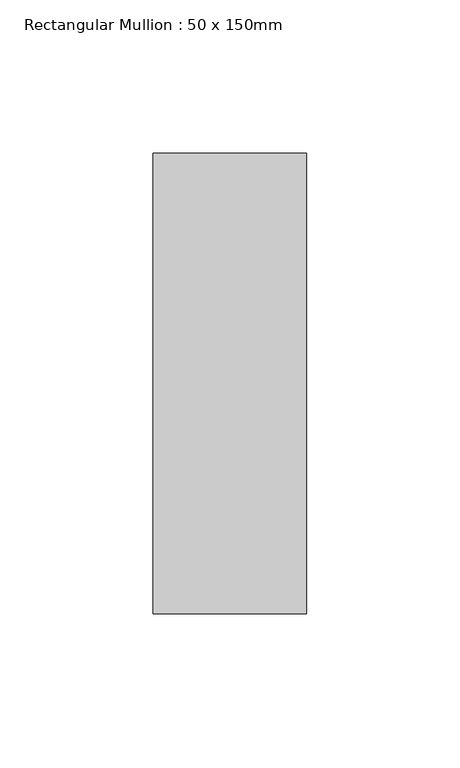
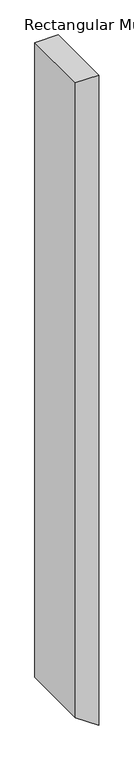
"""IFC4 building model written with IfcOpenShell, lengths in millimetres: member geometry, Rectangular Mullion : 50 x 150mm."""

from ifc_helpers import new_model, si_unit, frame, origin, place, context, project, spatial, polyline, outline, extrude, source, transform, mapped, element, save


def rectangular_mullion_50_x_150mm_93a95515(model_context):
    return source(origin(), model_context, "Body", "SweptSolid", [
        extrude(outline(polyline([(0.0, 25.0), (0.0, -25.0), (-1431.7258818, -25.0), (-1466.7362587, 25.0), (0.0, 25.0)])), frame((0.0, -75.0, 0.0), z_axis=(0.0, 1.0, 0.0), x_axis=(0.0, 0.0, 1.0)), (0.0, 0.0, 1.0), 150.0),
    ])


if __name__ == "__main__":
    model = new_model("IFC4")
    model_context = context("Model", 3, world=origin())
    ifc_project = project(units=[si_unit("LENGTHUNIT", "METRE", prefix="MILLI")], contexts=[model_context])
    site = spatial("IfcSite", under=ifc_project)
    building = spatial("IfcBuilding", under=site)
    placement = place(None, origin())
    rectangular_mullion_50_x_150mm_shape = rectangular_mullion_50_x_150mm_93a95515(model_context)
    element("IfcMember", 1, ObjectType="Rectangular Mullion : 50 x 150mm", at=placement, inside=building, context=model_context, shape_type="MappedRepresentation", body=[
        mapped(rectangular_mullion_50_x_150mm_shape, transform((0.0, 0.0, 0.0), x_axis=(1.0, 0.0, 0.0), y_axis=(0.0, 1.0, 0.0), z_axis=(0.0, 0.0, 1.0))),
    ])
    save(model, "model.ifc")

# Revit data of these elements
# Type "Rectangular Mullion : 50 x 150mm"
#   built-in parameter 1007304 = 0.492126 (stored number, unit not read)
#   built-in parameter 1007301 = 0.082021 (stored number, unit not read)
#   built-in parameter 1007300 = 0.082021 (stored number, unit not read)
# Element 1 (IfcMember, "Rectangular Mullion : 50 x 150mm")
#   Materials on its faces: "Aluminium"
# Materials
#   "Aluminium": class "Metal", colour RGB 247 247 247, transparency 0, Description = "Aluminium 6061", Cost = 0
